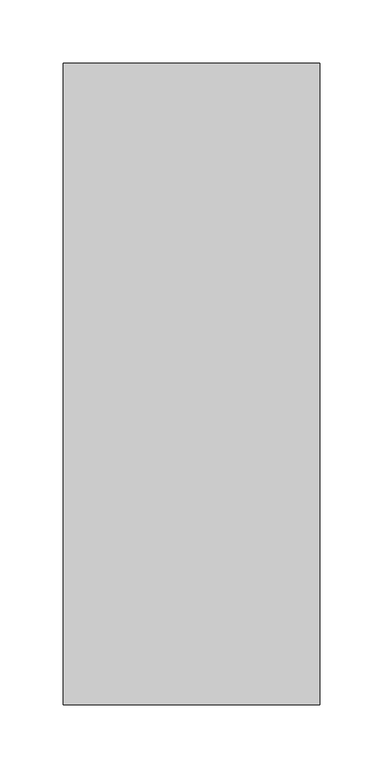
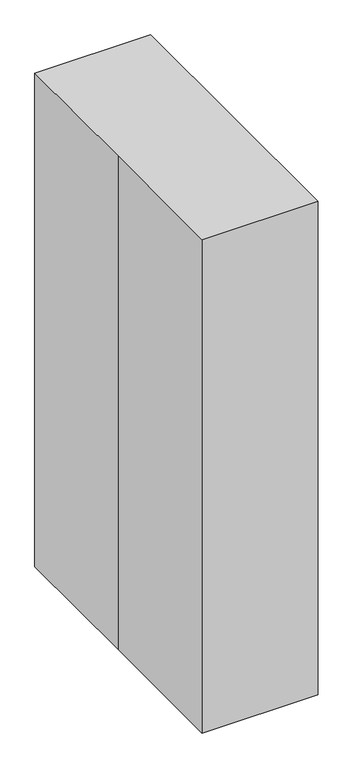
"""IFC4 building model written with IfcOpenShell, lengths in millimetres: proxy geometry, P1150 - Valve, Rinse, Bedpan, With Disinfectant Injector : P1150 - Valve, Rinse, Bedpan, With Disinfectant Injector."""

from ifc_helpers import new_model, si_unit, point, frame, frame_2d, origin, origin_with_axes, origin_2d, place, context, project, spatial, polyline, circle_curve, trimmed, segment, composite_curve, outline, extrude, source, transform, mapped, element, save


def specialty_equipment_394be24a(model_context):
    return source(origin(), model_context, "Body", "SweptSolid", [
        extrude(outline(composite_curve([segment(trimmed(circle_curve(frame_2d((0.0, 400.05)), 19.05), [point((19.05, 400.05))], [point((-19.05, 400.05))], False, "CARTESIAN"), True, "CONTINUOUS"), segment(trimmed(circle_curve(frame_2d((0.0, 400.05)), 19.05), [point((-19.05, 400.05))], [point((19.05, 400.05))], False, "CARTESIAN"), True, "CONTINUOUS")], self_intersect=False)), frame((26.9875, 0.0, 0.0), z_axis=(1.0, 0.0, 0.0), x_axis=(0.0, 1.0, 0.0)), (0.0, 0.0, 1.0), 25.4),
        extrude(outline(composite_curve([segment(trimmed(circle_curve(frame_2d((50.8, 39.6875)), 19.05), [point((50.8, 20.6375))], [point((50.8, 58.7375))], False, "CARTESIAN"), True, "CONTINUOUS"), segment(trimmed(circle_curve(frame_2d((50.8, 39.6875)), 19.05), [point((50.8, 58.7375))], [point((50.8, 20.6375))], False, "CARTESIAN"), True, "CONTINUOUS")], self_intersect=False)), frame((0.0, -25.4, 0.0), z_axis=(0.0, 1.0, 0.0), x_axis=(0.0, 0.0, 1.0)), (0.0, 0.0, 1.0), 50.8),
        extrude(outline(composite_curve([segment(trimmed(circle_curve(frame_2d((39.6875, 0.0)), 6.35), [point((33.3375, 0.0))], [point((46.0375, 0.0))], False, "CARTESIAN"), True, "CONTINUOUS"), segment(trimmed(circle_curve(frame_2d((39.6875, 0.0)), 6.35), [point((46.0375, 0.0))], [point((33.3375, 0.0))], False, "CARTESIAN"), True, "CONTINUOUS")], self_intersect=False)), frame((0.0, 0.0, 50.8), z_axis=(0.0, 0.0, 1.0), x_axis=(1.0, 0.0, 0.0)), (0.0, 0.0, 1.0), 349.25),
        extrude(outline(composite_curve([segment(trimmed(circle_curve(origin_2d(), 31.75), [point((-31.75, 0.0))], [point((31.75, 0.0))], False, "CARTESIAN"), True, "CONTINUOUS"), segment(trimmed(circle_curve(origin_2d(), 31.75), [point((31.75, 0.0))], [point((-31.75, 0.0))], False, "CARTESIAN"), True, "CONTINUOUS")], self_intersect=False), holes=[composite_curve([segment(trimmed(circle_curve(origin_2d(), 25.4), [point((-25.4, 0.0))], [point((25.4, 0.0))], True, "CARTESIAN"), True, "CONTINUOUS"), segment(trimmed(circle_curve(origin_2d(), 25.4), [point((25.4, 0.0))], [point((-25.4, 0.0))], True, "CARTESIAN"), True, "CONTINUOUS")], self_intersect=False)]), frame((0.0, 0.0, 25.4), z_axis=(0.0, 0.0, 1.0), x_axis=(1.0, 0.0, 0.0)), (0.0, 0.0, 1.0), 50.8),
        extrude(outline(polyline([(-101.6, -254.0), (-101.6, 0.0), (-101.6, 254.0), (101.6, 254.0), (101.6, -254.0), (-101.6, -254.0)])), origin_with_axes(), (0.0, 0.0, 1.0), 914.4),
    ])


if __name__ == "__main__":
    model = new_model("IFC4")
    model_context = context("Model", 3, world=origin())
    ifc_project = project(units=[si_unit("LENGTHUNIT", "METRE", prefix="MILLI")], contexts=[model_context])
    site = spatial("IfcSite", under=ifc_project)
    building = spatial("IfcBuilding", under=site)
    placement = place(None, origin())
    specialty_equipment_shape = specialty_equipment_394be24a(model_context)
    element("IfcBuildingElementProxy", 1, Name="P1150 - Valve, Rinse, Bedpan, With Disinfectant Injector : P1150 - Valve, Rinse, Bedpan, With Disinfectant Injector", ObjectType="P1150 - Valve, Rinse, Bedpan, With Disinfectant Injector : P1150 - Valve, Rinse, Bedpan, With Disinfectant Injector", at=placement, inside=building, context=model_context, shape_type="MappedRepresentation", body=[
        mapped(specialty_equipment_shape, transform((0.0, 0.0, 0.0), x_axis=(1.0, 0.0, 0.0), y_axis=(0.0, 1.0, 0.0), z_axis=(0.0, 0.0, 1.0))),
    ])
    save(model, "model.ifc")

# Revit data of these elements
# Type "P1150 - Valve, Rinse, Bedpan, With Disinfectant Injector : P1150 - Valve, Rinse, Bedpan, With Disinfectant Injector"
#   Watts2 = "0"
#   Watts1 = "0"
#   Unit_Issue = "EA"
#   UTIL_6_Misc = "-"
#   UTIL_5_NonMedGas = "-"
#   UTIL_4_MiscGas = "-"
#   UTIL_3_MedGas = "-"
#   UTIL_2_Elec = "-"
#   UTIL_1_WaterDrain = "J"
#   Nomenclature = "Valve, Rinse, Bedpan, With Disinfectant Injector"
#   NSN = "4510"
#   Location [instance default] = ""
#   JSN = "P1150"
#   Fund_Source_VA = "-"
#   Fund_Source_Navy = "-"
#   Fund_Source_Army = "-"
#   Fund_Source_AF = "-"
#   ELEC_Volts2 = "0"
#   ELEC_Volts1 = "0"
#   ELEC_Phase2 = "0"
#   ELEC_Phase1 = "0"
#   ELEC_HertzSwitch = "0"
#   ELEC_HertzDependent = "0"
#   ELEC_Hertz = "0"
#   ELEC_Amps2 = "0"
#   ELEC_Amps1 = "0"
#   DetailDescription = "Bedpan rinsing valve with deodorant/disinfectant spray. Unit is wall mounted above a water closet having an exposed flush valve. Flush water shall be available to rinse the pan with the balance used to flush the waste. Used in dirty utility rooms located in patient care areas throughout the hospital. Unit is used to flush and disinfect a dirty bedpan."
#   CAT_VA = "A"
#   CAT_Navy = "A"
#   CAT_IHS = "-"
#   CAT_Army = "A"
#   CAT_AF = "A"
#   BTUperhour = "0"
#   Weight_IP = 8
#   DIM_Width_IP = 0' - 8"
#   DIM_Height_IP = 3' - 0"
#   DIM_Depth_IP = 1' - 8"
# Element 1 (IfcBuildingElementProxy, "P1150 - Valve, Rinse, Bedpan, With Disinfectant Injector : P1150 - Valve, Rinse, Bedpan, With Disinfectant Injector")
#   Materials on its faces: "EquipSpace"
# Materials
#   "EquipSpace": class "Unassigned", colour RGB 221 217 195, transparency 0.5
